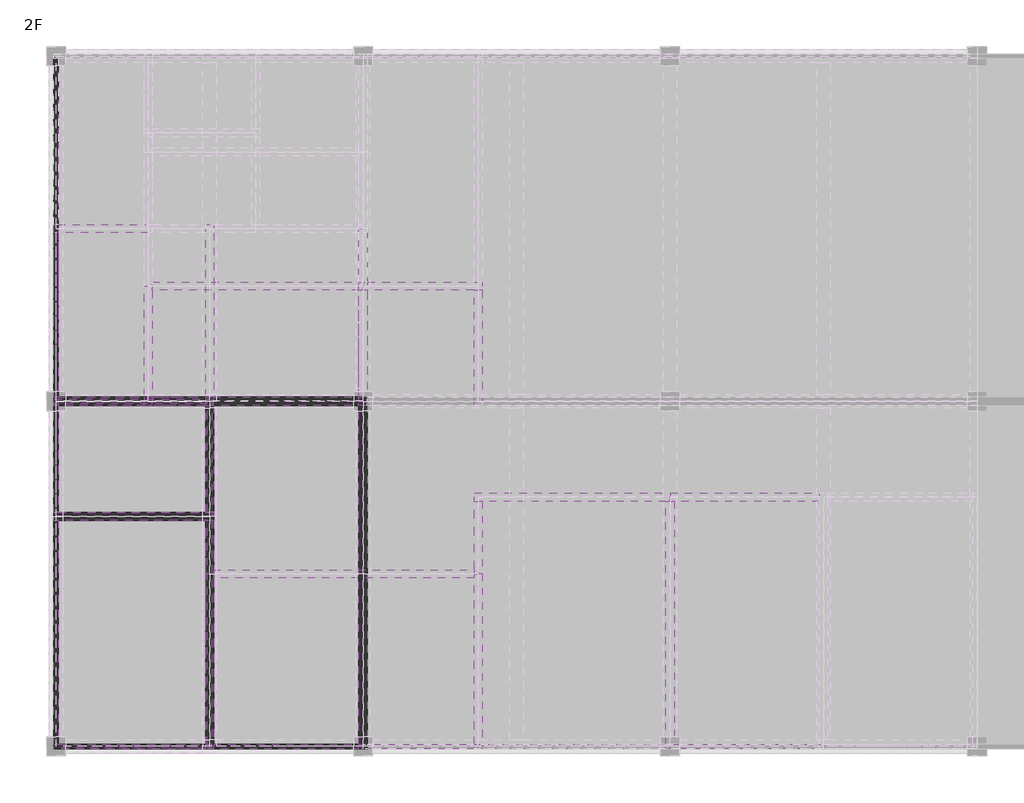
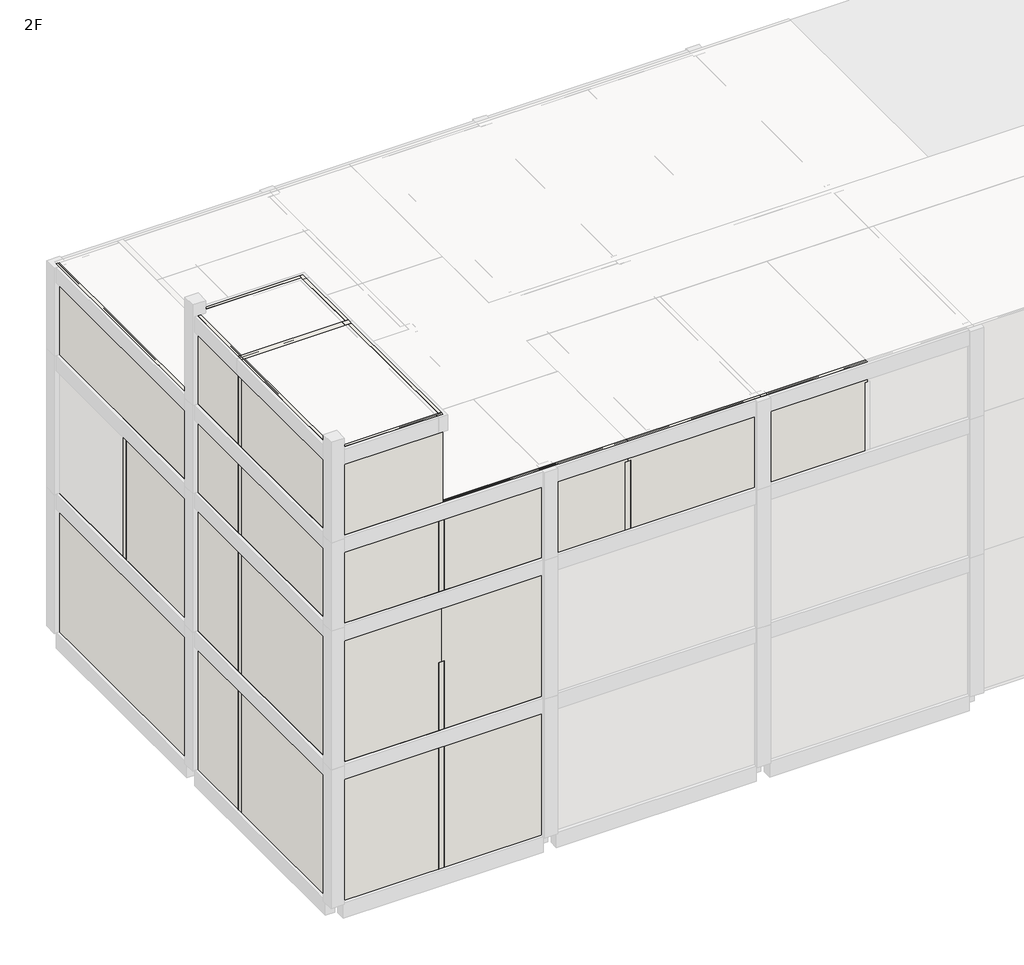
# One storey, part 1 of 7: 56 walls.
"""IFC4 building model written with IfcOpenShell, lengths in millimetres."""

from ifc_helpers import new_model, si_unit, frame, origin, place, context, project, spatial, polyline, outline, extrude, faceted_brep, element, save

model = new_model("IFC4")

# Units and contexts
model_context = context("Model", 3, world=origin())
ifc_project = project(units=[si_unit("LENGTHUNIT", "METRE", prefix="MILLI")], contexts=[model_context])

# Site, building, storey
site = spatial("IfcSite", under=ifc_project)
building = spatial("IfcBuilding", under=site)
storey = spatial("IfcBuildingStorey", under=building, Name="2F", Elevation=3500.0)

# Walls
placement = place(None, origin())
element("IfcWall", 1, ObjectType="WA211_Exterior-Cement Brick-90mm", at=placement, inside=storey, context=model_context, shape_type="SweptSolid", body=[
    extrude(outline(polyline([(45516.6521483, 181866.8614395), (45516.6521483, 173030.8614395), (45402.6521483, 173030.8614395), (45402.6521483, 181866.8614395), (45516.6521483, 181866.8614395)])), frame((0.0, 0.0, 3500.0), z_axis=(0.0, 0.0, 1.0), x_axis=(1.0, 0.0, 0.0)), (0.0, 0.0, 1.0), 5500.0),
])
element("IfcWall", 2, ObjectType="WA211_Exterior-Cement Brick-90mm", at=placement, inside=storey, context=model_context, shape_type="SweptSolid", body=[
    extrude(outline(polyline([(49566.6521483, 163980.8614395), (53352.6521483, 163980.8614395), (53352.6521483, 163866.8614395), (49566.6521483, 163866.8614395), (49566.6521483, 163980.8614395)])), frame((0.0, 0.0, 3500.0), z_axis=(0.0, 0.0, 1.0), x_axis=(1.0, 0.0, 0.0)), (0.0, 0.0, 1.0), 5500.0),
])
element("IfcWall", 3, ObjectType="WA211_Exterior-Cement Brick-90mm", at=placement, inside=storey, context=model_context, shape_type="SweptSolid", body=[
    extrude(outline(polyline([(45516.6521483, 172816.8614395), (45516.6521483, 170030.8614395), (45402.6521483, 170030.8614395), (45402.6521483, 172816.8614395), (45516.6521483, 172816.8614395)])), frame((0.0, 0.0, 3500.0), z_axis=(0.0, 0.0, 1.0), x_axis=(1.0, 0.0, 0.0)), (0.0, 0.0, 1.0), 5500.0),
])
element("IfcWall", 4, ObjectType="WA211_Exterior-Cement Brick-90mm", at=placement, inside=storey, context=model_context, shape_type="SweptSolid", body=[
    extrude(outline(polyline([(45516.6521483, 169816.8614395), (45516.6521483, 163980.8614395), (45402.6521483, 163980.8614395), (45402.6521483, 169816.8614395), (45516.6521483, 169816.8614395)])), frame((0.0, 0.0, 3500.0), z_axis=(0.0, 0.0, 1.0), x_axis=(1.0, 0.0, 0.0)), (0.0, 0.0, 1.0), 5500.0),
])
element("IfcWall", 5, ObjectType="WA211_Exterior-Cement Brick-90mm", at=placement, inside=storey, context=model_context, shape_type="Brep", body=[
    faceted_brep([(49352.6521483, 163980.8614395, 3500.0), (45516.6521483, 163980.8614395, 3500.0), (45402.6521483, 163980.8614395, 3500.0), (45402.6521483, 163980.8614395, 9000.0), (45516.6521483, 163980.8614395, 9000.0), (49352.6521483, 163980.8614395, 9000.0), (49352.6521483, 163866.8614395, 3500.0), (49352.6521483, 163866.8614395, 9000.0), (45402.6521483, 163866.8614395, 9000.0), (45402.6521483, 163866.8614395, 3500.0)], [[[0, 1, 2, 3, 4, 5]], [[6, 7, 8, 9]], [[2, 1, 0, 6, 9]], [[5, 4, 3, 8, 7]], [[0, 5, 7, 6]], [[3, 2, 9, 8]]]),
])
element("IfcWall", 6, ObjectType="WA211_Exterior-Cement Brick-90mm", at=placement, inside=storey, context=model_context, shape_type="SweptSolid", body=[
    extrude(outline(polyline([(45516.6521483, 177316.8614395), (45516.6521483, 173030.8614395), (45402.6521483, 173030.8614395), (45402.6521483, 177316.8614395), (45516.6521483, 177316.8614395)])), frame((0.0, 0.0, 9000.0), z_axis=(0.0, 0.0, 1.0), x_axis=(1.0, 0.0, 0.0)), (0.0, 0.0, 1.0), 5500.0),
])
element("IfcWall", 7, ObjectType="WA211_Exterior-Cement Brick-90mm", at=placement, inside=storey, context=model_context, shape_type="SweptSolid", body=[
    extrude(outline(polyline([(45516.6521483, 172816.8614395), (45516.6521483, 170030.8614395), (45402.6521483, 170030.8614395), (45402.6521483, 172816.8614395), (45516.6521483, 172816.8614395)])), frame((0.0, 0.0, 9000.0), z_axis=(0.0, 0.0, 1.0), x_axis=(1.0, 0.0, 0.0)), (0.0, 0.0, 1.0), 5500.0),
])
element("IfcWall", 8, ObjectType="WA211_Exterior-Cement Brick-90mm", at=placement, inside=storey, context=model_context, shape_type="SweptSolid", body=[
    extrude(outline(polyline([(45516.6521483, 169816.8614395), (45516.6521483, 163980.8614395), (45402.6521483, 163980.8614395), (45402.6521483, 169816.8614395), (45516.6521483, 169816.8614395)])), frame((0.0, 0.0, 9000.0), z_axis=(0.0, 0.0, 1.0), x_axis=(1.0, 0.0, 0.0)), (0.0, 0.0, 1.0), 5500.0),
])
element("IfcWall", 9, ObjectType="WA211_Exterior-Cement Brick-90mm", at=placement, inside=storey, context=model_context, shape_type="Brep", body=[
    faceted_brep([(49352.6521483, 163980.8614395, 9000.0), (45516.6521483, 163980.8614395, 9000.0), (45402.6521483, 163980.8614395, 9000.0), (45402.6521483, 163980.8614395, 14500.0), (45516.6521483, 163980.8614395, 14500.0), (49459.6521483, 163980.8614395, 14500.0), (49459.6521483, 163980.8614395, 11700.0), (49352.6521483, 163980.8614395, 11700.0), (49352.6521483, 163866.8614395, 9000.0), (49352.6521483, 163866.8614395, 11700.0), (49459.6521483, 163866.8614395, 11700.0), (49459.6521483, 163866.8614395, 14500.0), (45402.6521483, 163866.8614395, 14500.0), (45402.6521483, 163866.8614395, 9000.0)], [[[0, 1, 2, 3, 4, 5, 6, 7]], [[8, 9, 10, 11, 12, 13]], [[2, 1, 0, 8, 13]], [[5, 4, 3, 12, 11]], [[3, 2, 13, 12]], [[6, 5, 11, 10]], [[6, 10, 9, 7]], [[0, 7, 9, 8]]]),
])
element("IfcWall", 10, ObjectType="WA211_Exterior-Cement Brick-90mm", at=placement, inside=storey, context=model_context, shape_type="SweptSolid", body=[
    extrude(outline(polyline([(9000.0, 53352.6521483), (12000.0, 53352.6521483), (12000.0, 53459.6521483), (14500.0, 53459.6521483), (14500.0, 49459.6521483), (11700.0, 49459.6521483), (11700.0, 49566.6521483), (9000.0, 49566.6521483), (9000.0, 53352.6521483)])), frame((0.0, 163866.8614395, 0.0), z_axis=(0.0, 1.0, 0.0), x_axis=(0.0, 0.0, 1.0)), (0.0, 0.0, 1.0), 114.0),
])
element("IfcWall", 11, ObjectType="WA211_Exterior-Cement Brick-90mm", at=placement, inside=storey, context=model_context, shape_type="SweptSolid", body=[
    extrude(outline(polyline([(14500.0, 65352.6521483), (17200.0, 65352.6521483), (17200.0, 65459.6521483), (18000.0, 65459.6521483), (18000.0, 61459.6521483), (17200.0, 61459.6521483), (17200.0, 61566.6521483), (14500.0, 61566.6521483), (14500.0, 65352.6521483)])), frame((0.0, 163866.8614395, 0.0), z_axis=(0.0, 1.0, 0.0), x_axis=(0.0, 0.0, 1.0)), (0.0, 0.0, 1.0), 114.0),
])
element("IfcWall", 12, ObjectType="WA211_Exterior-Cement Brick-90mm", at=placement, inside=storey, context=model_context, shape_type="SweptSolid", body=[
    extrude(outline(polyline([(14500.0, 61352.6521483), (17200.0, 61352.6521483), (17200.0, 61459.6521483), (18000.0, 61459.6521483), (18000.0, 56459.6521483), (17200.0, 56459.6521483), (17200.0, 56566.6521483), (14500.0, 56566.6521483), (14500.0, 61352.6521483)])), frame((0.0, 163866.8614395, 0.0), z_axis=(0.0, 1.0, 0.0), x_axis=(0.0, 0.0, 1.0)), (0.0, 0.0, 1.0), 114.0),
])
element("IfcWall", 13, ObjectType="WA211_Exterior-Cement Brick-90mm", at=placement, inside=storey, context=model_context, shape_type="SweptSolid", body=[
    extrude(outline(polyline([(14500.0, 56352.6521483), (17200.0, 56352.6521483), (17200.0, 56459.6521483), (18000.0, 56459.6521483), (18000.0, 49566.6521483), (14500.0, 49566.6521483), (14500.0, 56352.6521483)])), frame((0.0, 163866.8614395, 0.0), z_axis=(0.0, 1.0, 0.0), x_axis=(0.0, 0.0, 1.0)), (0.0, 0.0, 1.0), 114.0),
])
element("IfcWall", 14, ObjectType="WA211_Exterior-Cement Brick-90mm", at=placement, inside=storey, context=model_context, shape_type="SweptSolid", body=[
    extrude(outline(polyline([(45516.6521483, 181866.8614395), (45516.6521483, 173030.8614395), (45402.6521483, 173030.8614395), (45402.6521483, 181866.8614395), (45516.6521483, 181866.8614395)])), frame((0.0, 0.0, 14500.0), z_axis=(0.0, 0.0, 1.0), x_axis=(1.0, 0.0, 0.0)), (0.0, 0.0, 1.0), 3500.0),
])
element("IfcWall", 15, ObjectType="WA211_Exterior-Cement Brick-90mm", at=placement, inside=storey, context=model_context, shape_type="SweptSolid", body=[
    extrude(outline(polyline([(45516.6521483, 172816.8614395), (45516.6521483, 170030.8614395), (45402.6521483, 170030.8614395), (45402.6521483, 172816.8614395), (45516.6521483, 172816.8614395)])), frame((0.0, 0.0, 14500.0), z_axis=(0.0, 0.0, 1.0), x_axis=(1.0, 0.0, 0.0)), (0.0, 0.0, 1.0), 3500.0),
])
element("IfcWall", 16, ObjectType="WA211_Exterior-Cement Brick-90mm", at=placement, inside=storey, context=model_context, shape_type="SweptSolid", body=[
    extrude(outline(polyline([(45516.6521483, 169816.8614395), (45516.6521483, 163980.8614395), (45402.6521483, 163980.8614395), (45402.6521483, 169816.8614395), (45516.6521483, 169816.8614395)])), frame((0.0, 0.0, 14500.0), z_axis=(0.0, 0.0, 1.0), x_axis=(1.0, 0.0, 0.0)), (0.0, 0.0, 1.0), 3500.0),
])
element("IfcWall", 17, ObjectType="WA211_Exterior-Cement Brick-90mm", at=placement, inside=storey, context=model_context, shape_type="Brep", body=[
    faceted_brep([(49352.6521483, 163980.8614395, 14500.0), (45516.6521483, 163980.8614395, 14500.0), (45402.6521483, 163980.8614395, 14500.0), (45402.6521483, 163980.8614395, 18000.0), (45516.6521483, 163980.8614395, 18000.0), (49352.6521483, 163980.8614395, 18000.0), (49352.6521483, 163866.8614395, 14500.0), (49352.6521483, 163866.8614395, 18000.0), (45402.6521483, 163866.8614395, 18000.0), (45402.6521483, 163866.8614395, 14500.0)], [[[0, 1, 2, 3, 4, 5]], [[6, 7, 8, 9]], [[2, 1, 0, 6, 9]], [[5, 4, 3, 8, 7]], [[0, 5, 7, 6]], [[3, 2, 9, 8]]]),
])
element("IfcWall", 18, ObjectType="WA211_Exterior-Cement Brick-90mm", at=placement, inside=storey, context=model_context, shape_type="Brep", body=[
    faceted_brep([(49402.6521483, 172980.8614395, 18000.0), (49402.6521483, 172866.8614395, 18000.0), (49402.6521483, 170030.8614395, 18000.0), (49402.6521483, 170030.8614395, 21500.0), (49402.6521483, 172866.8614395, 21500.0), (49402.6521483, 172980.8614395, 21500.0), (49516.6521483, 172980.8614395, 18000.0), (49516.6521483, 172980.8614395, 21500.0), (49516.6521483, 170030.8614395, 21500.0), (49516.6521483, 170030.8614395, 18000.0)], [[[0, 1, 2, 3, 4, 5]], [[6, 7, 8, 9]], [[2, 1, 0, 6, 9]], [[5, 4, 3, 8, 7]], [[0, 5, 7, 6]], [[3, 2, 9, 8]]]),
])
element("IfcWall", 19, ObjectType="WA211_Exterior-Cement Brick-90mm", at=placement, inside=storey, context=model_context, shape_type="SweptSolid", body=[
    extrude(outline(polyline([(45516.6521483, 172866.8614395), (45516.6521483, 170030.8614395), (45402.6521483, 170030.8614395), (45402.6521483, 172866.8614395), (45516.6521483, 172866.8614395)])), frame((0.0, 0.0, 18000.0), z_axis=(0.0, 0.0, 1.0), x_axis=(1.0, 0.0, 0.0)), (0.0, 0.0, 1.0), 3500.0),
])
element("IfcWall", 20, ObjectType="WA211_Exterior-Cement Brick-90mm", at=placement, inside=storey, context=model_context, shape_type="Brep", body=[
    faceted_brep([(45402.6521483, 172866.8614395, 18000.0), (45516.6521483, 172866.8614395, 18000.0), (49402.6521483, 172866.8614395, 18000.0), (49402.6521483, 172866.8614395, 21500.0), (45516.6521483, 172866.8614395, 21500.0), (45402.6521483, 172866.8614395, 21500.0), (45402.6521483, 172980.8614395, 18000.0), (45402.6521483, 172980.8614395, 21500.0), (49402.6521483, 172980.8614395, 21500.0), (49402.6521483, 172980.8614395, 18000.0)], [[[0, 1, 2, 3, 4, 5]], [[6, 7, 8, 9]], [[2, 1, 0, 6, 9]], [[5, 4, 3, 8, 7]], [[0, 5, 7, 6]], [[3, 2, 9, 8]]]),
])
element("IfcWall", 21, ObjectType="WA211_Exterior-Cement Brick-90mm", at=placement, inside=storey, context=model_context, shape_type="SweptSolid", body=[
    extrude(outline(polyline([(45516.6521483, 169816.8614395), (45516.6521483, 163980.8614395), (45402.6521483, 163980.8614395), (45402.6521483, 169816.8614395), (45516.6521483, 169816.8614395)])), frame((0.0, 0.0, 18000.0), z_axis=(0.0, 0.0, 1.0), x_axis=(1.0, 0.0, 0.0)), (0.0, 0.0, 1.0), 3500.0),
])
element("IfcWall", 22, ObjectType="WA211_Exterior-Cement Brick-90mm", at=placement, inside=storey, context=model_context, shape_type="Brep", body=[
    faceted_brep([(49516.6521483, 163980.8614395, 18000.0), (49402.6521483, 163980.8614395, 18000.0), (45516.6521483, 163980.8614395, 18000.0), (45402.6521483, 163980.8614395, 18000.0), (45402.6521483, 163980.8614395, 21500.0), (45516.6521483, 163980.8614395, 21500.0), (49402.6521483, 163980.8614395, 21500.0), (49516.6521483, 163980.8614395, 21500.0), (49516.6521483, 163866.8614395, 18000.0), (49516.6521483, 163866.8614395, 21500.0), (45402.6521483, 163866.8614395, 21500.0), (45402.6521483, 163866.8614395, 18000.0)], [[[0, 1, 2, 3, 4, 5, 6, 7]], [[8, 9, 10, 11]], [[3, 2, 1, 0, 8, 11]], [[7, 6, 5, 4, 10, 9]], [[0, 7, 9, 8]], [[4, 3, 11, 10]]]),
])
element("IfcWall", 23, ObjectType="WA211_Exterior-Cement Brick-90mm", at=placement, inside=storey, context=model_context, shape_type="SweptSolid", body=[
    extrude(outline(polyline([(49402.6521483, 163980.8614395), (49402.6521483, 169816.8614395), (49516.6521483, 169816.8614395), (49516.6521483, 163980.8614395), (49402.6521483, 163980.8614395)])), frame((0.0, 0.0, 18000.0), z_axis=(0.0, 0.0, 1.0), x_axis=(1.0, 0.0, 0.0)), (0.0, 0.0, 1.0), 3500.0),
])
element("IfcWall", 24, ObjectType="WA221_Interior-Cement Block-190mm", at=placement, inside=storey, context=model_context, shape_type="SweptSolid", body=[
    extrude(outline(polyline([(49566.6521483, 173030.8614395), (53352.6521483, 173030.8614395), (53352.6521483, 172816.8614395), (49566.6521483, 172816.8614395), (49566.6521483, 173030.8614395)])), frame((0.0, 0.0, 3500.0), z_axis=(0.0, 0.0, 1.0), x_axis=(1.0, 0.0, 0.0)), (0.0, 0.0, 1.0), 5500.0),
])
element("IfcWall", 25, ObjectType="WA221_Interior-Cement Block-190mm", at=placement, inside=storey, context=model_context, shape_type="Brep", body=[
    faceted_brep([(45402.6521483, 172816.8614395, 3500.0), (45516.6521483, 172816.8614395, 3500.0), (49352.6521483, 172816.8614395, 3500.0), (49352.6521483, 172816.8614395, 9000.0), (45516.6521483, 172816.8614395, 9000.0), (45402.6521483, 172816.8614395, 9000.0), (45402.6521483, 173030.8614395, 3500.0), (45402.6521483, 173030.8614395, 9000.0), (45516.6521483, 173030.8614395, 9000.0), (49352.6521483, 173030.8614395, 9000.0), (49352.6521483, 173030.8614395, 3500.0), (45516.6521483, 173030.8614395, 3500.0)], [[[0, 1, 2, 3, 4, 5]], [[6, 7, 8, 9, 10, 11]], [[2, 1, 0, 6, 11, 10]], [[5, 4, 3, 9, 8, 7]], [[0, 5, 7, 6]], [[3, 2, 10, 9]]]),
])
element("IfcWall", 26, ObjectType="WA221_Interior-Cement Block-190mm", at=placement, inside=storey, context=model_context, shape_type="Brep", body=[
    faceted_brep([(53566.6521483, 163866.8614395, 3500.0), (53566.6521483, 163980.8614395, 3500.0), (53566.6521483, 172816.8614395, 3500.0), (53566.6521483, 173030.8614395, 3500.0), (53566.6521483, 173030.8614395, 9000.0), (53566.6521483, 172816.8614395, 9000.0), (53566.6521483, 163980.8614395, 9000.0), (53566.6521483, 163866.8614395, 9000.0), (53352.6521483, 163866.8614395, 3500.0), (53352.6521483, 163866.8614395, 9000.0), (53352.6521483, 163980.8614395, 9000.0), (53352.6521483, 172816.8614395, 9000.0), (53352.6521483, 173030.8614395, 9000.0), (53352.6521483, 173030.8614395, 3500.0), (53352.6521483, 172816.8614395, 3500.0), (53352.6521483, 163980.8614395, 3500.0)], [[[0, 1, 2, 3, 4, 5, 6, 7]], [[8, 9, 10, 11, 12, 13, 14, 15]], [[3, 2, 1, 0, 8, 15, 14, 13]], [[7, 6, 5, 4, 12, 11, 10, 9]], [[0, 7, 9, 8]], [[4, 3, 13, 12]]]),
])
element("IfcWall", 27, ObjectType="WA221_Interior-Cement Block-190mm", at=placement, inside=storey, context=model_context, shape_type="Brep", body=[
    faceted_brep([(49352.6521483, 173030.8614395, 3500.0), (49352.6521483, 172816.8614395, 3500.0), (49352.6521483, 170030.8614395, 3500.0), (49352.6521483, 170030.8614395, 9000.0), (49352.6521483, 172816.8614395, 9000.0), (49352.6521483, 173030.8614395, 9000.0), (49566.6521483, 173030.8614395, 3500.0), (49566.6521483, 173030.8614395, 9000.0), (49566.6521483, 172816.8614395, 9000.0), (49566.6521483, 170030.8614395, 9000.0), (49566.6521483, 170030.8614395, 3500.0), (49566.6521483, 172816.8614395, 3500.0)], [[[0, 1, 2, 3, 4, 5]], [[6, 7, 8, 9, 10, 11]], [[2, 1, 0, 6, 11, 10]], [[5, 4, 3, 9, 8, 7]], [[0, 5, 7, 6]], [[3, 2, 10, 9]]]),
])
element("IfcWall", 28, ObjectType="WA221_Interior-Cement Block-190mm", at=placement, inside=storey, context=model_context, shape_type="Brep", body=[
    faceted_brep([(49352.6521483, 169816.8614395, 3500.0), (49352.6521483, 163980.8614395, 3500.0), (49352.6521483, 163866.8614395, 3500.0), (49352.6521483, 163866.8614395, 9000.0), (49352.6521483, 163980.8614395, 9000.0), (49352.6521483, 169816.8614395, 9000.0), (49566.6521483, 169816.8614395, 3500.0), (49566.6521483, 169816.8614395, 9000.0), (49566.6521483, 163980.8614395, 9000.0), (49566.6521483, 163866.8614395, 9000.0), (49566.6521483, 163866.8614395, 3500.0), (49566.6521483, 163980.8614395, 3500.0)], [[[0, 1, 2, 3, 4, 5]], [[6, 7, 8, 9, 10, 11]], [[2, 1, 0, 6, 11, 10]], [[5, 4, 3, 9, 8, 7]], [[3, 2, 10, 9]], [[0, 5, 7, 6]]]),
])
element("IfcWall", 29, ObjectType="WA221_Interior-Cement Block-190mm", at=placement, inside=storey, context=model_context, shape_type="Brep", body=[
    faceted_brep([(45402.6521483, 169816.8614395, 3500.0), (45516.6521483, 169816.8614395, 3500.0), (49352.6521483, 169816.8614395, 3500.0), (49566.6521483, 169816.8614395, 3500.0), (49566.6521483, 169816.8614395, 9000.0), (49352.6521483, 169816.8614395, 9000.0), (45516.6521483, 169816.8614395, 9000.0), (45402.6521483, 169816.8614395, 9000.0), (45402.6521483, 170030.8614395, 3500.0), (45402.6521483, 170030.8614395, 9000.0), (45516.6521483, 170030.8614395, 9000.0), (49352.6521483, 170030.8614395, 9000.0), (49566.6521483, 170030.8614395, 9000.0), (49566.6521483, 170030.8614395, 3500.0), (49352.6521483, 170030.8614395, 3500.0), (45516.6521483, 170030.8614395, 3500.0)], [[[0, 1, 2, 3, 4, 5, 6, 7]], [[8, 9, 10, 11, 12, 13, 14, 15]], [[3, 2, 1, 0, 8, 15, 14, 13]], [[7, 6, 5, 4, 12, 11, 10, 9]], [[0, 7, 9, 8]], [[4, 3, 13, 12]]]),
])
element("IfcWall", 30, ObjectType="WA221_Interior-Cement Block-190mm", at=placement, inside=storey, context=model_context, shape_type="Brep", body=[
    faceted_brep([(53566.6521483, 172923.8614395, 9000.0), (53566.6521483, 173030.8614395, 9000.0), (53566.6521483, 177316.8614395, 9000.0), (53566.6521483, 177316.8614395, 11700.0), (53566.6521483, 177423.8614395, 11700.0), (53566.6521483, 177423.8614395, 12400.0), (53566.6521483, 173030.8614395, 12400.0), (53566.6521483, 172816.8614395, 12400.0), (53566.6521483, 172816.8614395, 12000.0), (53566.6521483, 172923.8614395, 12000.0), (53352.6521483, 172923.8614395, 9000.0), (53352.6521483, 172923.8614395, 12000.0), (53352.6521483, 172816.8614395, 12000.0), (53352.6521483, 172816.8614395, 12400.0), (53352.6521483, 177423.8614395, 12400.0), (53352.6521483, 177423.8614395, 11700.0), (53352.6521483, 177316.8614395, 11700.0), (53352.6521483, 177316.8614395, 9000.0)], [[[0, 1, 2, 3, 4, 5, 6, 7, 8, 9]], [[10, 11, 12, 13, 14, 15, 16, 17]], [[2, 1, 0, 10, 17]], [[7, 6, 5, 14, 13]], [[0, 9, 11, 10]], [[8, 12, 11, 9]], [[8, 7, 13, 12]], [[5, 4, 15, 14]], [[15, 4, 3, 16]], [[3, 2, 17, 16]]]),
])
element("IfcWall", 31, ObjectType="WA221_Interior-Cement Block-190mm", at=placement, inside=storey, context=model_context, shape_type="Brep", body=[
    faceted_brep([(53566.6521483, 163866.8614395, 9000.0), (53566.6521483, 163980.8614395, 9000.0), (53566.6521483, 172816.8614395, 9000.0), (53566.6521483, 172923.8614395, 9000.0), (53566.6521483, 172923.8614395, 12000.0), (53566.6521483, 172816.8614395, 12000.0), (53566.6521483, 163980.8614395, 12000.0), (53566.6521483, 163866.8614395, 12000.0), (53352.6521483, 163866.8614395, 9000.0), (53352.6521483, 163866.8614395, 12000.0), (53352.6521483, 163980.8614395, 12000.0), (53352.6521483, 172816.8614395, 12000.0), (53352.6521483, 172923.8614395, 12000.0), (53352.6521483, 172923.8614395, 9000.0), (53352.6521483, 163980.8614395, 9000.0), (53459.6521483, 163866.8614395, 12000.0)], [[[0, 1, 2, 3, 4, 5, 6, 7]], [[8, 9, 10, 11, 12, 13, 14]], [[3, 2, 1, 0, 8, 14, 13]], [[4, 3, 13, 12]], [[7, 6, 5, 4, 12, 11, 10, 9, 15]], [[0, 7, 15, 9, 8]]]),
])
element("IfcWall", 32, ObjectType="WA221_Interior-Cement Block-190mm", at=placement, inside=storey, context=model_context, shape_type="Brep", body=[
    faceted_brep([(47859.6521483, 177530.8614395, 9000.0), (47752.6521483, 177530.8614395, 9000.0), (45516.6521483, 177530.8614395, 9000.0), (45402.6521483, 177530.8614395, 9000.0), (45402.6521483, 177530.8614395, 14500.0), (45516.6521483, 177530.8614395, 14500.0), (47752.6521483, 177530.8614395, 14500.0), (47966.6521483, 177530.8614395, 14500.0), (47966.6521483, 177530.8614395, 11700.0), (47859.6521483, 177530.8614395, 11700.0), (47859.6521483, 177316.8614395, 9000.0), (47859.6521483, 177316.8614395, 11700.0), (47966.6521483, 177316.8614395, 11700.0), (47966.6521483, 177316.8614395, 14500.0), (45516.6521483, 177316.8614395, 14500.0), (45402.6521483, 177316.8614395, 14500.0), (45402.6521483, 177316.8614395, 9000.0), (45516.6521483, 177316.8614395, 9000.0)], [[[0, 1, 2, 3, 4, 5, 6, 7, 8, 9]], [[10, 11, 12, 13, 14, 15, 16, 17]], [[3, 2, 1, 0, 10, 17, 16]], [[7, 6, 5, 4, 15, 14, 13]], [[0, 9, 11, 10]], [[8, 12, 11, 9]], [[8, 7, 13, 12]], [[4, 3, 16, 15]]]),
])
element("IfcWall", 33, ObjectType="WA221_Interior-Cement Block-190mm", at=placement, inside=storey, context=model_context, shape_type="Brep", body=[
    faceted_brep([(45402.6521483, 172816.8614395, 9000.0), (45516.6521483, 172816.8614395, 9000.0), (49352.6521483, 172816.8614395, 9000.0), (49566.6521483, 172816.8614395, 9000.0), (49566.6521483, 172816.8614395, 14500.0), (49352.6521483, 172816.8614395, 14500.0), (45516.6521483, 172816.8614395, 14500.0), (45402.6521483, 172816.8614395, 14500.0), (45402.6521483, 173030.8614395, 9000.0), (45402.6521483, 173030.8614395, 14500.0), (45516.6521483, 173030.8614395, 14500.0), (49566.6521483, 173030.8614395, 14500.0), (49566.6521483, 173030.8614395, 11700.0), (49566.6521483, 173030.8614395, 9000.0), (49352.6521483, 173030.8614395, 9000.0), (45516.6521483, 173030.8614395, 9000.0)], [[[0, 1, 2, 3, 4, 5, 6, 7]], [[8, 9, 10, 11, 12, 13, 14, 15]], [[3, 2, 1, 0, 8, 15, 14, 13]], [[7, 6, 5, 4, 11, 10, 9]], [[0, 7, 9, 8]], [[3, 13, 12, 11, 4]]]),
])
element("IfcWall", 34, ObjectType="WA221_Interior-Cement Block-190mm", at=placement, inside=storey, context=model_context, shape_type="Brep", body=[
    faceted_brep([(49352.6521483, 177530.8614395, 9000.0), (49352.6521483, 177316.8614395, 9000.0), (49352.6521483, 173030.8614395, 9000.0), (49352.6521483, 173030.8614395, 11700.0), (49352.6521483, 177316.8614395, 11700.0), (49352.6521483, 177530.8614395, 11700.0), (49566.6521483, 177530.8614395, 9000.0), (49566.6521483, 177530.8614395, 11700.0), (49566.6521483, 177316.8614395, 11700.0), (49566.6521483, 173030.8614395, 11700.0), (49566.6521483, 173030.8614395, 9000.0), (49566.6521483, 177316.8614395, 9000.0)], [[[0, 1, 2, 3, 4, 5]], [[6, 7, 8, 9, 10, 11]], [[2, 1, 0, 6, 11, 10]], [[5, 4, 3, 9, 8, 7]], [[0, 5, 7, 6]], [[3, 2, 10, 9]]]),
])
element("IfcWall", 35, ObjectType="WA221_Interior-Cement Block-190mm", at=placement, inside=storey, context=model_context, shape_type="Brep", body=[
    faceted_brep([(49566.6521483, 170030.8614395, 14500.0), (49566.6521483, 170030.8614395, 9000.0), (49352.6521483, 170030.8614395, 9000.0), (45516.6521483, 170030.8614395, 9000.0), (45402.6521483, 170030.8614395, 9000.0), (45402.6521483, 170030.8614395, 14500.0), (45516.6521483, 170030.8614395, 14500.0), (49352.6521483, 170030.8614395, 14500.0), (49566.6521483, 169816.8614395, 9000.0), (49566.6521483, 169816.8614395, 11700.0), (49566.6521483, 169816.8614395, 14500.0), (45516.6521483, 169816.8614395, 14500.0), (45402.6521483, 169816.8614395, 14500.0), (45402.6521483, 169816.8614395, 9000.0), (45516.6521483, 169816.8614395, 9000.0), (49352.6521483, 169816.8614395, 9000.0)], [[[0, 1, 2, 3, 4, 5, 6, 7]], [[8, 9, 10, 11, 12, 13, 14, 15]], [[4, 3, 2, 1, 8, 15, 14, 13]], [[0, 7, 6, 5, 12, 11, 10]], [[5, 4, 13, 12]], [[0, 10, 9, 8, 1]]]),
])
element("IfcWall", 36, ObjectType="WA221_Interior-Cement Block-190mm", at=placement, inside=storey, context=model_context, shape_type="SweptSolid", body=[
    extrude(outline(polyline([(49352.6521483, 170030.8614395), (49352.6521483, 172816.8614395), (49566.6521483, 172816.8614395), (49566.6521483, 170030.8614395), (49352.6521483, 170030.8614395)])), frame((0.0, 0.0, 9000.0), z_axis=(0.0, 0.0, 1.0), x_axis=(1.0, 0.0, 0.0)), (0.0, 0.0, 1.0), 5500.0),
])
element("IfcWall", 37, ObjectType="WA221_Interior-Cement Block-190mm", at=placement, inside=storey, context=model_context, shape_type="Brep", body=[
    faceted_brep([(49352.6521483, 169816.8614395, 9000.0), (49352.6521483, 163980.8614395, 9000.0), (49352.6521483, 163866.8614395, 9000.0), (49352.6521483, 163866.8614395, 11700.0), (49352.6521483, 163980.8614395, 11700.0), (49352.6521483, 169816.8614395, 11700.0), (49566.6521483, 169816.8614395, 9000.0), (49566.6521483, 169816.8614395, 11700.0), (49566.6521483, 163980.8614395, 11700.0), (49566.6521483, 163866.8614395, 11700.0), (49566.6521483, 163866.8614395, 9000.0), (49566.6521483, 163980.8614395, 9000.0), (49459.6521483, 163866.8614395, 11700.0)], [[[0, 1, 2, 3, 4, 5]], [[6, 7, 8, 9, 10, 11]], [[2, 1, 0, 6, 11, 10]], [[5, 4, 3, 12, 9, 8, 7]], [[0, 5, 7, 6]], [[3, 2, 10, 9, 12]]]),
])
element("IfcWall", 38, ObjectType="WA221_Interior-Cement Block-190mm", at=placement, inside=storey, context=model_context, shape_type="Brep", body=[
    faceted_brep([(61352.6521483, 170316.8614395, 14500.0), (61352.6521483, 163980.8614395, 14500.0), (61352.6521483, 163866.8614395, 14500.0), (61352.6521483, 163866.8614395, 17200.0), (61352.6521483, 163980.8614395, 17200.0), (61352.6521483, 170316.8614395, 17200.0), (61566.6521483, 170316.8614395, 14500.0), (61566.6521483, 170316.8614395, 17200.0), (61566.6521483, 163980.8614395, 17200.0), (61566.6521483, 163866.8614395, 17200.0), (61566.6521483, 163866.8614395, 14500.0), (61566.6521483, 163980.8614395, 14500.0), (61459.6521483, 170316.8614395, 14500.0), (61459.6521483, 163866.8614395, 17200.0), (61459.6521483, 170316.8614395, 17200.0)], [[[0, 1, 2, 3, 4, 5]], [[6, 7, 8, 9, 10, 11]], [[2, 1, 0, 12, 6, 11, 10]], [[5, 4, 3, 13, 9, 8, 7, 14]], [[3, 2, 10, 9, 13]], [[0, 5, 14, 7, 6, 12]]]),
])
element("IfcWall", 39, ObjectType="WA221_Interior-Cement Block-190mm", at=placement, inside=storey, context=model_context, shape_type="Brep", body=[
    faceted_brep([(61459.6521483, 170316.8614395, 14500.0), (61566.6521483, 170316.8614395, 14500.0), (65352.6521483, 170316.8614395, 14500.0), (65352.6521483, 170316.8614395, 17200.0), (61566.6521483, 170316.8614395, 17200.0), (61459.6521483, 170316.8614395, 17200.0), (61459.6521483, 170530.8614395, 14500.0), (61459.6521483, 170530.8614395, 17200.0), (65352.6521483, 170530.8614395, 17200.0), (65352.6521483, 170530.8614395, 14500.0)], [[[0, 1, 2, 3, 4, 5]], [[6, 7, 8, 9]], [[2, 1, 0, 6, 9]], [[5, 4, 3, 8, 7]], [[0, 5, 7, 6]], [[3, 2, 9, 8]]]),
])
element("IfcWall", 40, ObjectType="WA221_Interior-Cement Block-190mm", at=placement, inside=storey, context=model_context, shape_type="Brep", body=[
    faceted_brep([(56566.6521483, 172816.8614395, 14500.0), (56566.6521483, 173030.8614395, 14500.0), (56566.6521483, 175816.8614395, 14500.0), (56566.6521483, 175816.8614395, 17200.0), (56566.6521483, 173030.8614395, 17200.0), (56566.6521483, 172816.8614395, 17200.0), (56352.6521483, 172816.8614395, 14500.0), (56352.6521483, 172816.8614395, 17200.0), (56352.6521483, 175816.8614395, 17200.0), (56352.6521483, 175816.8614395, 14500.0)], [[[0, 1, 2, 3, 4, 5]], [[6, 7, 8, 9]], [[2, 1, 0, 6, 9]], [[5, 4, 3, 8, 7]], [[0, 5, 7, 6]], [[3, 2, 9, 8]]]),
])
element("IfcWall", 41, ObjectType="WA221_Interior-Cement Block-190mm", at=placement, inside=storey, context=model_context, shape_type="Brep", body=[
    faceted_brep([(56566.6521483, 163866.8614395, 14500.0), (56566.6521483, 163980.8614395, 14500.0), (56566.6521483, 168423.8614395, 14500.0), (56566.6521483, 168423.8614395, 17200.0), (56566.6521483, 163980.8614395, 17200.0), (56566.6521483, 163866.8614395, 17200.0), (56352.6521483, 163866.8614395, 14500.0), (56352.6521483, 163866.8614395, 17200.0), (56352.6521483, 163980.8614395, 17200.0), (56352.6521483, 168316.8614395, 17200.0), (56352.6521483, 168423.8614395, 17200.0), (56352.6521483, 168423.8614395, 14500.0), (56352.6521483, 168316.8614395, 14500.0), (56352.6521483, 163980.8614395, 14500.0), (56459.6521483, 163866.8614395, 17200.0)], [[[0, 1, 2, 3, 4, 5]], [[6, 7, 8, 9, 10, 11, 12, 13]], [[2, 1, 0, 6, 13, 12, 11]], [[3, 2, 11, 10]], [[5, 4, 3, 10, 9, 8, 7, 14]], [[0, 5, 14, 7, 6]]]),
])
element("IfcWall", 42, ObjectType="WA221_Interior-Cement Block-190mm", at=placement, inside=storey, context=model_context, shape_type="Brep", body=[
    faceted_brep([(56352.6521483, 170316.8614395, 14500.0), (56566.6521483, 170316.8614395, 14500.0), (61352.6521483, 170316.8614395, 14500.0), (61459.6521483, 170316.8614395, 14500.0), (61459.6521483, 170316.8614395, 17200.0), (61352.6521483, 170316.8614395, 17200.0), (56566.6521483, 170316.8614395, 17200.0), (56352.6521483, 170316.8614395, 17200.0), (56352.6521483, 170530.8614395, 14500.0), (56352.6521483, 170530.8614395, 17200.0), (61459.6521483, 170530.8614395, 17200.0), (61459.6521483, 170530.8614395, 14500.0)], [[[0, 1, 2, 3, 4, 5, 6, 7]], [[8, 9, 10, 11]], [[3, 2, 1, 0, 8, 11]], [[4, 3, 11, 10]], [[7, 6, 5, 4, 10, 9]], [[0, 7, 9, 8]]]),
])
element("IfcWall", 43, ObjectType="WA221_Interior-Cement Block-190mm", at=placement, inside=storey, context=model_context, shape_type="Brep", body=[
    faceted_brep([(56566.6521483, 168423.8614395, 14500.0), (56566.6521483, 170316.8614395, 14500.0), (56566.6521483, 170316.8614395, 17200.0), (56566.6521483, 168423.8614395, 17200.0), (56352.6521483, 168423.8614395, 14500.0), (56352.6521483, 168423.8614395, 17200.0), (56352.6521483, 168530.8614395, 17200.0), (56352.6521483, 170316.8614395, 17200.0), (56352.6521483, 170316.8614395, 14500.0), (56352.6521483, 168530.8614395, 14500.0)], [[[0, 1, 2, 3]], [[4, 5, 6, 7, 8, 9]], [[1, 0, 4, 9, 8]], [[3, 2, 7, 6, 5]], [[0, 3, 5, 4]], [[2, 1, 8, 7]]]),
])
element("IfcWall", 44, ObjectType="WA221_Interior-Cement Block-190mm", at=placement, inside=storey, context=model_context, shape_type="Brep", body=[
    faceted_brep([(49352.6521483, 168423.8614395, 18000.0), (49352.6521483, 168423.8614395, 14500.0), (49352.6521483, 163980.8614395, 14500.0), (49352.6521483, 163866.8614395, 14500.0), (49352.6521483, 163866.8614395, 18000.0), (49352.6521483, 163980.8614395, 18000.0), (49566.6521483, 168423.8614395, 14500.0), (49566.6521483, 168423.8614395, 18000.0), (49566.6521483, 163980.8614395, 18000.0), (49566.6521483, 163866.8614395, 18000.0), (49566.6521483, 163866.8614395, 14500.0), (49566.6521483, 163980.8614395, 14500.0), (49566.6521483, 168316.8614395, 14500.0)], [[[0, 1, 2, 3, 4, 5]], [[6, 7, 8, 9, 10, 11, 12]], [[3, 2, 1, 6, 12, 11, 10]], [[0, 5, 4, 9, 8, 7]], [[0, 7, 6, 1]], [[4, 3, 10, 9]]]),
])
element("IfcWall", 45, ObjectType="WA221_Interior-Cement Block-190mm", at=placement, inside=storey, context=model_context, shape_type="Brep", body=[
    faceted_brep([(56352.6521483, 168530.8614395, 14500.0), (49566.6521483, 168530.8614395, 14500.0), (49566.6521483, 168530.8614395, 17200.0), (56352.6521483, 168530.8614395, 17200.0), (56352.6521483, 168316.8614395, 14500.0), (56352.6521483, 168316.8614395, 17200.0), (49566.6521483, 168316.8614395, 17200.0), (49566.6521483, 168316.8614395, 14500.0), (56352.6521483, 168423.8614395, 14500.0), (49566.6521483, 168423.8614395, 14500.0), (56352.6521483, 168423.8614395, 17200.0)], [[[0, 1, 2, 3]], [[4, 5, 6, 7]], [[1, 0, 8, 4, 7, 9]], [[3, 2, 6, 5, 10]], [[0, 3, 10, 5, 4, 8]], [[2, 1, 9, 7, 6]]]),
])
element("IfcWall", 46, ObjectType="WA221_Interior-Cement Block-190mm", at=placement, inside=storey, context=model_context, shape_type="Brep", body=[
    faceted_brep([(47966.6521483, 175816.8614395, 14500.0), (53352.6521483, 175816.8614395, 14500.0), (53459.6521483, 175816.8614395, 14500.0), (53459.6521483, 175816.8614395, 17200.0), (53352.6521483, 175816.8614395, 17200.0), (47966.6521483, 175816.8614395, 17200.0), (47966.6521483, 176030.8614395, 14500.0), (47966.6521483, 176030.8614395, 17200.0), (53352.6521483, 176030.8614395, 17200.0), (53459.6521483, 176030.8614395, 17200.0), (53459.6521483, 176030.8614395, 14500.0), (53352.6521483, 176030.8614395, 14500.0), (47966.6521483, 175923.8614395, 14500.0)], [[[0, 1, 2, 3, 4, 5]], [[6, 7, 8, 9, 10, 11]], [[2, 1, 0, 12, 6, 11, 10]], [[3, 2, 10, 9]], [[5, 4, 3, 9, 8, 7]], [[0, 5, 7, 6, 12]]]),
])
element("IfcWall", 47, ObjectType="WA221_Interior-Cement Block-190mm", at=placement, inside=storey, context=model_context, shape_type="Brep", body=[
    faceted_brep([(53459.6521483, 175816.8614395, 14500.0), (53566.6521483, 175816.8614395, 14500.0), (56352.6521483, 175816.8614395, 14500.0), (56566.6521483, 175816.8614395, 14500.0), (56566.6521483, 175816.8614395, 17200.0), (56352.6521483, 175816.8614395, 17200.0), (53566.6521483, 175816.8614395, 17200.0), (53459.6521483, 175816.8614395, 17200.0), (53459.6521483, 176030.8614395, 14500.0), (53459.6521483, 176030.8614395, 17200.0), (53566.6521483, 176030.8614395, 17200.0), (56352.6521483, 176030.8614395, 17200.0), (56566.6521483, 176030.8614395, 17200.0), (56566.6521483, 176030.8614395, 14500.0), (56352.6521483, 176030.8614395, 14500.0), (53566.6521483, 176030.8614395, 14500.0)], [[[0, 1, 2, 3, 4, 5, 6, 7]], [[8, 9, 10, 11, 12, 13, 14, 15]], [[3, 2, 1, 0, 8, 15, 14, 13]], [[7, 6, 5, 4, 12, 11, 10, 9]], [[0, 7, 9, 8]], [[4, 3, 13, 12]]]),
])
element("IfcWall", 48, ObjectType="WA221_Interior-Cement Block-190mm", at=placement, inside=storey, context=model_context, shape_type="Brep", body=[
    faceted_brep([(47752.6521483, 175923.8614395, 18000.0), (47752.6521483, 175923.8614395, 14500.0), (47752.6521483, 173030.8614395, 14500.0), (47752.6521483, 172816.8614395, 14500.0), (47752.6521483, 172816.8614395, 18000.0), (47752.6521483, 173030.8614395, 18000.0), (47966.6521483, 175923.8614395, 14500.0), (47966.6521483, 175923.8614395, 18000.0), (47966.6521483, 173030.8614395, 18000.0), (47966.6521483, 172816.8614395, 18000.0), (47966.6521483, 172816.8614395, 14500.0), (47966.6521483, 173030.8614395, 14500.0), (47966.6521483, 175816.8614395, 14500.0)], [[[0, 1, 2, 3, 4, 5]], [[6, 7, 8, 9, 10, 11, 12]], [[3, 2, 1, 6, 12, 11, 10]], [[0, 5, 4, 9, 8, 7]], [[0, 7, 6, 1]], [[4, 3, 10, 9]]]),
])
element("IfcWall", 49, ObjectType="WA221_Interior-Cement Block-190mm", at=placement, inside=storey, context=model_context, shape_type="SweptSolid", body=[
    extrude(outline(polyline([(49352.6521483, 172816.8614395), (47966.6521483, 172816.8614395), (47966.6521483, 173030.8614395), (49352.6521483, 173030.8614395), (49352.6521483, 172816.8614395)])), frame((0.0, 0.0, 14500.0), z_axis=(0.0, 0.0, 1.0), x_axis=(1.0, 0.0, 0.0)), (0.0, 0.0, 1.0), 3500.0),
])
element("IfcWall", 50, ObjectType="WA221_Interior-Cement Block-190mm", at=placement, inside=storey, context=model_context, shape_type="Brep", body=[
    faceted_brep([(53566.6521483, 173030.8614395, 14500.0), (53352.6521483, 173030.8614395, 14500.0), (49566.6521483, 173030.8614395, 14500.0), (49566.6521483, 173030.8614395, 17200.0), (53352.6521483, 173030.8614395, 17200.0), (53566.6521483, 173030.8614395, 17200.0), (53566.6521483, 172816.8614395, 14500.0), (53566.6521483, 172816.8614395, 17200.0), (49566.6521483, 172816.8614395, 17200.0), (49566.6521483, 172816.8614395, 14500.0)], [[[0, 1, 2, 3, 4, 5]], [[6, 7, 8, 9]], [[2, 1, 0, 6, 9]], [[5, 4, 3, 8, 7]], [[0, 5, 7, 6]], [[3, 2, 9, 8]]]),
])
element("IfcWall", 51, ObjectType="WA221_Interior-Cement Block-190mm", at=placement, inside=storey, context=model_context, shape_type="Brep", body=[
    faceted_brep([(53352.6521483, 175816.8614395, 14500.0), (53352.6521483, 173030.8614395, 14500.0), (53352.6521483, 173030.8614395, 17200.0), (53352.6521483, 175816.8614395, 17200.0), (53566.6521483, 175816.8614395, 14500.0), (53566.6521483, 175816.8614395, 17200.0), (53566.6521483, 173030.8614395, 17200.0), (53566.6521483, 173030.8614395, 14500.0), (53459.6521483, 175816.8614395, 14500.0), (53459.6521483, 175816.8614395, 17200.0)], [[[0, 1, 2, 3]], [[4, 5, 6, 7]], [[1, 0, 8, 4, 7]], [[3, 2, 6, 5, 9]], [[0, 3, 9, 5, 4, 8]], [[2, 1, 7, 6]]]),
])
element("IfcWall", 52, ObjectType="WA221_Interior-Cement Block-190mm", at=placement, inside=storey, context=model_context, shape_type="Brep", body=[
    faceted_brep([(47752.6521483, 173030.8614395, 14500.0), (45516.6521483, 173030.8614395, 14500.0), (45402.6521483, 173030.8614395, 14500.0), (45402.6521483, 173030.8614395, 18000.0), (45516.6521483, 173030.8614395, 18000.0), (47752.6521483, 173030.8614395, 18000.0), (47752.6521483, 172816.8614395, 14500.0), (47752.6521483, 172816.8614395, 18000.0), (45516.6521483, 172816.8614395, 18000.0), (45402.6521483, 172816.8614395, 18000.0), (45402.6521483, 172816.8614395, 14500.0), (45516.6521483, 172816.8614395, 14500.0)], [[[0, 1, 2, 3, 4, 5]], [[6, 7, 8, 9, 10, 11]], [[2, 1, 0, 6, 11, 10]], [[5, 4, 3, 9, 8, 7]], [[0, 5, 7, 6]], [[3, 2, 10, 9]]]),
])
element("IfcWall", 53, ObjectType="WA221_Interior-Cement Block-190mm", at=placement, inside=storey, context=model_context, shape_type="Brep", body=[
    faceted_brep([(45402.6521483, 169816.8614395, 14500.0), (45516.6521483, 169816.8614395, 14500.0), (49352.6521483, 169816.8614395, 14500.0), (49566.6521483, 169816.8614395, 14500.0), (49566.6521483, 169816.8614395, 18000.0), (49352.6521483, 169816.8614395, 18000.0), (45516.6521483, 169816.8614395, 18000.0), (45402.6521483, 169816.8614395, 18000.0), (45402.6521483, 170030.8614395, 14500.0), (45402.6521483, 170030.8614395, 18000.0), (45516.6521483, 170030.8614395, 18000.0), (49352.6521483, 170030.8614395, 18000.0), (49566.6521483, 170030.8614395, 18000.0), (49566.6521483, 170030.8614395, 14500.0), (49352.6521483, 170030.8614395, 14500.0), (45516.6521483, 170030.8614395, 14500.0)], [[[0, 1, 2, 3, 4, 5, 6, 7]], [[8, 9, 10, 11, 12, 13, 14, 15]], [[3, 2, 1, 0, 8, 15, 14, 13]], [[7, 6, 5, 4, 12, 11, 10, 9]], [[0, 7, 9, 8]], [[4, 3, 13, 12]]]),
])
element("IfcWall", 54, ObjectType="WA221_Interior-Cement Block-190mm", at=placement, inside=storey, context=model_context, shape_type="Brep", body=[
    faceted_brep([(49352.6521483, 173030.8614395, 18000.0), (49352.6521483, 173030.8614395, 14500.0), (49352.6521483, 172816.8614395, 14500.0), (49352.6521483, 170030.8614395, 14500.0), (49352.6521483, 170030.8614395, 18000.0), (49352.6521483, 172816.8614395, 18000.0), (49566.6521483, 173030.8614395, 14500.0), (49566.6521483, 173030.8614395, 17200.0), (49566.6521483, 173030.8614395, 18000.0), (49566.6521483, 170030.8614395, 18000.0), (49566.6521483, 170030.8614395, 14500.0), (49566.6521483, 172816.8614395, 14500.0)], [[[0, 1, 2, 3, 4, 5]], [[6, 7, 8, 9, 10, 11]], [[3, 2, 1, 6, 11, 10]], [[0, 5, 4, 9, 8]], [[4, 3, 10, 9]], [[0, 8, 7, 6, 1]]]),
])
element("IfcWall", 55, ObjectType="WA221_Interior-Cement Block-190mm", at=placement, inside=storey, context=model_context, shape_type="Brep", body=[
    faceted_brep([(49352.6521483, 169816.8614395, 14500.0), (49352.6521483, 168423.8614395, 14500.0), (49352.6521483, 168423.8614395, 18000.0), (49352.6521483, 169816.8614395, 18000.0), (49566.6521483, 169816.8614395, 14500.0), (49566.6521483, 169816.8614395, 18000.0), (49566.6521483, 168423.8614395, 18000.0), (49566.6521483, 168423.8614395, 14500.0), (49566.6521483, 168530.8614395, 14500.0)], [[[0, 1, 2, 3]], [[4, 5, 6, 7, 8]], [[1, 0, 4, 8, 7]], [[3, 2, 6, 5]], [[1, 7, 6, 2]], [[0, 3, 5, 4]]]),
])
element("IfcWall", 56, ObjectType="WA221_Interior-Cement Block-190mm", at=placement, inside=storey, context=model_context, shape_type="Brep", body=[
    faceted_brep([(49516.6521483, 170030.8614395, 18000.0), (49402.6521483, 170030.8614395, 18000.0), (45516.6521483, 170030.8614395, 18000.0), (45402.6521483, 170030.8614395, 18000.0), (45402.6521483, 170030.8614395, 21500.0), (45516.6521483, 170030.8614395, 21500.0), (49402.6521483, 170030.8614395, 21500.0), (49516.6521483, 170030.8614395, 21500.0), (49516.6521483, 169816.8614395, 18000.0), (49516.6521483, 169816.8614395, 21500.0), (49402.6521483, 169816.8614395, 21500.0), (45516.6521483, 169816.8614395, 21500.0), (45402.6521483, 169816.8614395, 21500.0), (45402.6521483, 169816.8614395, 18000.0), (45516.6521483, 169816.8614395, 18000.0), (49402.6521483, 169816.8614395, 18000.0)], [[[0, 1, 2, 3, 4, 5, 6, 7]], [[8, 9, 10, 11, 12, 13, 14, 15]], [[3, 2, 1, 0, 8, 15, 14, 13]], [[7, 6, 5, 4, 12, 11, 10, 9]], [[4, 3, 13, 12]], [[0, 7, 9, 8]]]),
])

save(model, "model.ifc")

# Revit data of these elements
# Type "WA211_Exterior-Cement Brick-90mm"
#   Type Comments = ""
#   Layers, outside or top first: 0 mm "A04AL081-00001_Skirt_Acrylic Emulsion Paint" (function 100); 0 mm "A04AL077-00001_Ext Wall Painting_Acrylic Emulsion Paint" (function 100); 12 mm "A04AS164-00001_Plastering_Ext" (function 4); 90 mm "A04AK073-00001_Concrete Brick_0.5B" (function 1); 12 mm "A04AS164-00002_Plastering_Int" (function 5); 0 mm "A04AL078-00002_Int Wall Painting_Water Emulsion Paint" (function 100); 0 mm "A04AL081-00001_Skirt_Acrylic Emulsion Paint" (function 100)
# Type "WA221_Interior-Cement Block-190mm"
#   Type Comments = ""
#   Layers, outside or top first: 0 mm "A04AL081-00001_Skirt_Acrylic Emulsion Paint" (function 100); 0 mm "A04AL078-00002_Int Wall Painting_Water Emulsion Paint" (function 100); 12 mm "A04AS164-00002_Plastering_Int" (function 2); 190 mm "A04AK069-00002_Reinforced Concrete Block_THK 100-200mm" (function 1); 12 mm "A04AS164-00002_Plastering_Int" (function 2); 0 mm "A04AL078-00002_Int Wall Painting_Water Emulsion Paint" (function 100); 0 mm "A04AL081-00001_Skirt_Acrylic Emulsion Paint" (function 100)
# Elements 1, 2, 3, 4 (IfcWall, "WA211_Exterior-Cement Brick-90mm")
#   Top Offset = 0 mm
#   Base Offset = 0 mm
#   Unconnected Height = 5500 mm
#   wall height = 5500 mm
#   Phase Created = New Construction
#   Base Constraint = 2F
#   Materials on its faces: "Default Wall", "A04AS164-00002_Plastering_Int", "A04AS164-00001_Plastering_Ext"
# Element 5 (IfcWall, "WA211_Exterior-Cement Brick-90mm")
#   Top Offset = 0 mm
#   Base Offset = 0 mm
#   Unconnected Height = 5500 mm
#   wall height = 5500 mm
#   Phase Created = New Construction
#   Base Constraint = 2F
#   Materials on its faces: "Default Wall", "A04AS164-00001_Plastering_Ext", "A04AS164-00002_Plastering_Int"
# Elements 6, 7, 8, 10 (IfcWall, "WA211_Exterior-Cement Brick-90mm")
#   Top Offset = 0 mm
#   Base Offset = 0 mm
#   Unconnected Height = 5500 mm
#   wall height = 5500 mm
#   Phase Created = New Construction
#   Base Constraint = 3F
#   Materials on its faces: "Default Wall", "A04AS164-00002_Plastering_Int", "A04AS164-00001_Plastering_Ext"
# Element 9 (IfcWall, "WA211_Exterior-Cement Brick-90mm")
#   Top Offset = 0 mm
#   Base Offset = 0 mm
#   Unconnected Height = 5500 mm
#   wall height = 5500 mm
#   Phase Created = New Construction
#   Base Constraint = 3F
#   Materials on its faces: "Default Wall", "A04AS164-00001_Plastering_Ext", "A04AS164-00002_Plastering_Int"
# Elements 11, 12, 13, 14, 15, 16 (IfcWall, "WA211_Exterior-Cement Brick-90mm")
#   Top Offset = 0 mm
#   Base Offset = 0 mm
#   Unconnected Height = 3500 mm
#   wall height = 3500 mm
#   Phase Created = New Construction
#   Base Constraint = 4F
#   Materials on its faces: "Default Wall", "A04AS164-00002_Plastering_Int", "A04AS164-00001_Plastering_Ext"
# Element 17 (IfcWall, "WA211_Exterior-Cement Brick-90mm")
#   Top Offset = 0 mm
#   Base Offset = 0 mm
#   Unconnected Height = 3500 mm
#   wall height = 3500 mm
#   Phase Created = New Construction
#   Base Constraint = 4F
#   Materials on its faces: "Default Wall", "A04AS164-00001_Plastering_Ext", "A04AS164-00002_Plastering_Int"
# Elements 18, 20 (IfcWall, "WA211_Exterior-Cement Brick-90mm")
#   Top Offset = 0 mm
#   Base Offset = 0 mm
#   Unconnected Height = 3500 mm
#   wall height = 3500 mm
#   Phase Created = New Construction
#   Base Constraint = PF
#   Materials on its faces: "Default Wall", "A04AS164-00001_Plastering_Ext", "A04AS164-00002_Plastering_Int"
# Elements 19, 21, 23 (IfcWall, "WA211_Exterior-Cement Brick-90mm")
#   Top Offset = 0 mm
#   Base Offset = 0 mm
#   Unconnected Height = 3500 mm
#   wall height = 3500 mm
#   Phase Created = New Construction
#   Base Constraint = PF
#   Materials on its faces: "Default Wall", "A04AS164-00002_Plastering_Int", "A04AS164-00001_Plastering_Ext"
# Element 22 (IfcWall, "WA211_Exterior-Cement Brick-90mm")
#   Top Offset = 0 mm
#   Base Offset = 0 mm
#   Unconnected Height = 3500 mm
#   wall height = 3500 mm
#   Phase Created = New Construction
#   Base Constraint = PF
#   Materials on its faces: "A04AS164-00001_Plastering_Ext", "Default Wall", "A04AS164-00002_Plastering_Int"
# Element 24 (IfcWall, "WA221_Interior-Cement Block-190mm")
#   Top Offset = 0 mm
#   Base Offset = 0 mm
#   Unconnected Height = 5500 mm
#   wall height = 5500 mm
#   Phase Created = New Construction
#   Base Constraint = 2F
#   Materials on its faces: "Default Wall", "A04AS164-00002_Plastering_Int"
# Elements 25, 28 (IfcWall, "WA221_Interior-Cement Block-190mm")
#   Top Offset = 0 mm
#   Base Offset = 0 mm
#   Unconnected Height = 5500 mm
#   wall height = 5500 mm
#   Phase Created = New Construction
#   Base Constraint = 2F
#   Materials on its faces: "Default Wall", "A04AS164-00002_Plastering_Int", "A04AS164-00001_Plastering_Ext"
# Elements 26, 29 (IfcWall, "WA221_Interior-Cement Block-190mm")
#   Top Offset = 0 mm
#   Base Offset = 0 mm
#   Unconnected Height = 5500 mm
#   wall height = 5500 mm
#   Phase Created = New Construction
#   Base Constraint = 2F
#   Materials on its faces: "A04AS164-00002_Plastering_Int", "Default Wall", "A04AS164-00001_Plastering_Ext"
# Element 27 (IfcWall, "WA221_Interior-Cement Block-190mm")
#   Top Offset = 0 mm
#   Base Offset = 0 mm
#   Unconnected Height = 5500 mm
#   wall height = 5500 mm
#   Phase Created = New Construction
#   Base Constraint = 2F
#   Materials on its faces: "A04AS164-00002_Plastering_Int", "Default Wall"
# Element 30 (IfcWall, "WA221_Interior-Cement Block-190mm")
#   Top Offset = 0 mm
#   Base Offset = 0 mm
#   Unconnected Height = 3400 mm
#   wall height = 3400 mm
#   Phase Created = New Construction
#   Base Constraint = 3F
#   Materials on its faces: "Default Wall", "A04AS164-00002_Plastering_Int"
# Element 31 (IfcWall, "WA221_Interior-Cement Block-190mm")
#   Top Offset = 0 mm
#   Base Offset = 0 mm
#   Unconnected Height = 3000 mm
#   wall height = 3000 mm
#   Phase Created = New Construction
#   Base Constraint = 3F
#   Materials on its faces: "Default Wall", "A04AS164-00002_Plastering_Int", "A04AS164-00001_Plastering_Ext"
# Element 32 (IfcWall, "WA221_Interior-Cement Block-190mm")
#   Top Offset = 0 mm
#   Base Offset = 0 mm
#   Unconnected Height = 5500 mm
#   wall height = 5500 mm
#   Phase Created = New Construction
#   Base Constraint = 3F
#   Materials on its faces: "Default Wall", "A04AS164-00002_Plastering_Int", "A04AS164-00001_Plastering_Ext"
# Elements 33, 35 (IfcWall, "WA221_Interior-Cement Block-190mm")
#   Top Offset = 0 mm
#   Base Offset = 0 mm
#   Unconnected Height = 5500 mm
#   wall height = 5500 mm
#   Phase Created = New Construction
#   Base Constraint = 3F
#   Materials on its faces: "A04AS164-00002_Plastering_Int", "Default Wall", "A04AS164-00001_Plastering_Ext"
# Element 34 (IfcWall, "WA221_Interior-Cement Block-190mm")
#   Top Offset = 0 mm
#   Base Offset = 0 mm
#   Unconnected Height = 2700 mm
#   wall height = 2700 mm
#   Phase Created = New Construction
#   Base Constraint = 3F
#   Materials on its faces: "A04AS164-00002_Plastering_Int", "Default Wall"
# Element 36 (IfcWall, "WA221_Interior-Cement Block-190mm")
#   Top Offset = 0 mm
#   Base Offset = 0 mm
#   Unconnected Height = 5500 mm
#   wall height = 5500 mm
#   Phase Created = New Construction
#   Base Constraint = 3F
#   Materials on its faces: "Default Wall", "A04AS164-00002_Plastering_Int"
# Element 37 (IfcWall, "WA221_Interior-Cement Block-190mm")
#   Top Offset = 0 mm
#   Base Offset = 0 mm
#   Unconnected Height = 2700 mm
#   wall height = 2700 mm
#   Phase Created = New Construction
#   Base Constraint = 3F
#   Materials on its faces: "Default Wall", "A04AS164-00002_Plastering_Int", "A04AS164-00001_Plastering_Ext"
# Elements 38, 41 (IfcWall, "WA221_Interior-Cement Block-190mm")
#   Top Offset = 0 mm
#   Base Offset = 0 mm
#   Unconnected Height = 2700 mm
#   wall height = 2700 mm
#   Phase Created = New Construction
#   Base Constraint = 4F
#   Materials on its faces: "Default Wall", "A04AS164-00002_Plastering_Int", "A04AS164-00001_Plastering_Ext"
# Elements 39, 43, 45, 46, 51 (IfcWall, "WA221_Interior-Cement Block-190mm")
#   Top Offset = 0 mm
#   Base Offset = 0 mm
#   Unconnected Height = 2700 mm
#   wall height = 2700 mm
#   Phase Created = New Construction
#   Base Constraint = 4F
#   Materials on its faces: "Default Wall", "A04AS164-00002_Plastering_Int"
# Elements 40, 42, 47, 50 (IfcWall, "WA221_Interior-Cement Block-190mm")
#   Top Offset = 0 mm
#   Base Offset = 0 mm
#   Unconnected Height = 2700 mm
#   wall height = 2700 mm
#   Phase Created = New Construction
#   Base Constraint = 4F
#   Materials on its faces: "A04AS164-00002_Plastering_Int", "Default Wall"
# Elements 44, 52 (IfcWall, "WA221_Interior-Cement Block-190mm")
#   Top Offset = 0 mm
#   Base Offset = 0 mm
#   Unconnected Height = 3500 mm
#   wall height = 3500 mm
#   Phase Created = New Construction
#   Base Constraint = 4F
#   Materials on its faces: "Default Wall", "A04AS164-00002_Plastering_Int", "A04AS164-00001_Plastering_Ext"
# Elements 48, 54 (IfcWall, "WA221_Interior-Cement Block-190mm")
#   Top Offset = 0 mm
#   Base Offset = 0 mm
#   Unconnected Height = 3500 mm
#   wall height = 3500 mm
#   Phase Created = New Construction
#   Base Constraint = 4F
#   Materials on its faces: "A04AS164-00002_Plastering_Int", "Default Wall"
# Elements 49, 55 (IfcWall, "WA221_Interior-Cement Block-190mm")
#   Top Offset = 0 mm
#   Base Offset = 0 mm
#   Unconnected Height = 3500 mm
#   wall height = 3500 mm
#   Phase Created = New Construction
#   Base Constraint = 4F
#   Materials on its faces: "Default Wall", "A04AS164-00002_Plastering_Int"
# Element 53 (IfcWall, "WA221_Interior-Cement Block-190mm")
#   Top Offset = 0 mm
#   Base Offset = 0 mm
#   Unconnected Height = 3500 mm
#   wall height = 3500 mm
#   Phase Created = New Construction
#   Base Constraint = 4F
#   Materials on its faces: "A04AS164-00002_Plastering_Int", "Default Wall", "A04AS164-00001_Plastering_Ext"
# Element 56 (IfcWall, "WA221_Interior-Cement Block-190mm")
#   Top Offset = 0 mm
#   Base Offset = 0 mm
#   Unconnected Height = 3500 mm
#   wall height = 3500 mm
#   Phase Created = New Construction
#   Base Constraint = PF
#   Materials on its faces: "A04AS164-00002_Plastering_Int", "Default Wall", "A04AS164-00001_Plastering_Ext"
# Materials
#   "A04AL081-00001_Skirt_Acrylic Emulsion Paint": class "Finish", colour RGB 128 128 64, transparency 0, Description = "Plastic", W00) Work Master Code = "A04AL081-00001", W01) Work Master_Lv1 = "Finishing Work", W02) Work Master_Lv2 = "Painting Work", W03) Work Master_Spec.1 = "Skirt Painting", W04) Work Master_Spec.2 = "Acrylic Emulsion Paint", W05) Work Master_Spec.3 = "100mm≤H<150mm", Cost = 0
#   "A04AL077-00001_Ext Wall Painting_Acrylic Emulsion Paint": class "Finish", colour RGB 128 128 64, transparency 0, Description = "Plastic", W00) Work Master Code = "A04AL077-00001", W01) Work Master_Lv1 = "Finishing Work", W02) Work Master_Lv2 = "Painting Work", W03) Work Master_Spec.1 = "External Wall Painting", W04) Work Master_Spec.2 = "Acrylic Emulsion Paint", Cost = 0
#   "A04AS164-00001_Plastering_Ext": class "Concrete", colour RGB 183 186 184, transparency 0, W00) Work Master Code = "A04AS164-00001", W01) Work Master_Lv1 = "Finishing Work", W02) Work Master_Lv2 = "Plastering Work", W03) Work Master_Spec.1 = "Plastering", W04) Work Master_Spec.2 = "for External Masonry Wall", Cost = 0
#   "A04AK073-00001_Concrete Brick_0.5B": class "Concrete", colour RGB 180 180 180, transparency 0, Description = "Conc. Block", W00) Work Master Code = "A04AK073-00001", W01) Work Master_Lv1 = "Finishing Work", W02) Work Master_Lv2 = "Masonry Work", W03) Work Master_Spec.1 = "Concrete Brick", W04) Work Master_Spec.2 = "[0.5B] w/ All Reinf.(Lath, Steel Tie, Anchor Bar, Mortar, ETC.), Filler, Sealant, Lintel/Sill for Opening, ETC.", Cost = 0
#   "A04AS164-00002_Plastering_Int": class "Concrete", colour RGB 183 186 184, transparency 0, Description = "LATEX PAINT ON THK.15 CEMENT PLASTER", W00) Work Master Code = "A04AS164-00002", W01) Work Master_Lv1 = "Finishing Work", W02) Work Master_Lv2 = "Plastering Work", W03) Work Master_Spec.1 = "Plastering", W04) Work Master_Spec.2 = "for Internal Masonry Wall", Cost = 0
#   "A04AL078-00002_Int Wall Painting_Water Emulsion Paint": class "Finish", colour RGB 128 128 64, transparency 0, Description = "Plastic", W00) Work Master Code = "A04AL078-00002", W01) Work Master_Lv1 = "Finishing Work", W02) Work Master_Lv2 = "Painting Work", W03) Work Master_Spec.1 = "Internal Wall Painting", W04) Work Master_Spec.2 = "Water Emulsion Paint", Cost = 0
